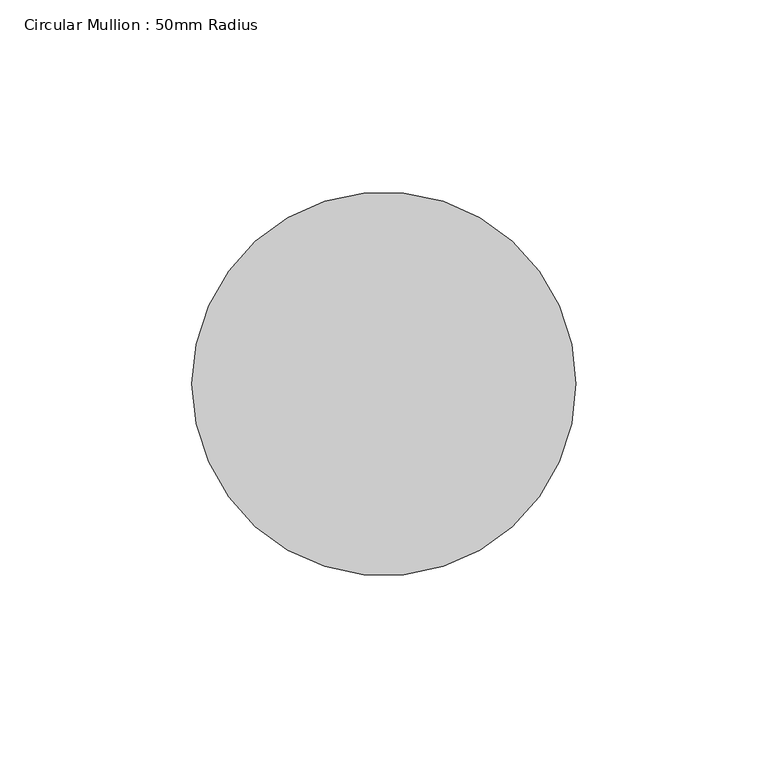
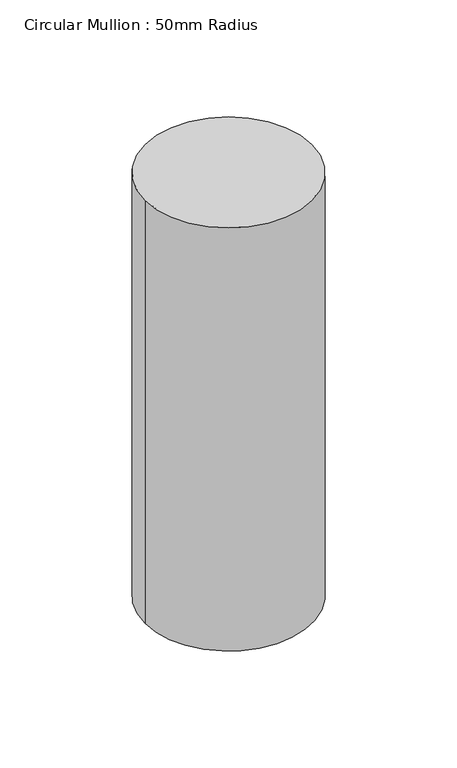
"""IFC4 building model written with IfcOpenShell, lengths in millimetres: member geometry, Circular Mullion : 50mm Radius."""

import ifcopenshell
import ifcopenshell.guid

model = None  # the IFC model being written
_history = None  # IfcOwnerHistory: only IFC2X3 demands one
_inside = {}  # id of a spatial element -> (the spatial element, [elements in it])
_under = {}  # id of a project, library or spatial element -> (it, [spatial elements below it])
_declared = {}  # id of a project -> (the project, [libraries it declares])
_typed = {}  # id of a type object -> (the type object, [elements of that type])
_made_of = {}  # id of a material, layer set ... -> (it, [elements and type objects made of it])


def new_model(schema):
    """Start an empty IFC model of exactly this schema.

    Asked for "IFC4X3", IfcOpenShell would pick the latest addendum, in which some entities
    have other attributes; the version numbers below select the first issue.
    IFC2X3 requires an IfcOwnerHistory on every rooted entity: one is made here for all.
    """
    global model, _history
    if schema == "IFC4X3":
        model = ifcopenshell.file(schema_version=(4, 3, 0, 0))
    else:
        model = ifcopenshell.file(schema=schema)
    _inside.clear()
    _under.clear()
    _declared.clear()
    _typed.clear()
    _made_of.clear()
    _history = None
    if model.schema == "IFC2X3":
        org = make("IfcOrganization", Name="unknown")
        user = make(
            "IfcPersonAndOrganization",
            ThePerson=make("IfcPerson", FamilyName="unknown"),
            TheOrganization=org,
        )
        app = make(
            "IfcApplication",
            ApplicationDeveloper=org,
            Version="unknown",
            ApplicationFullName="unknown",
            ApplicationIdentifier="unknown",
        )
        _history = make(
            "IfcOwnerHistory",
            OwningUser=user,
            OwningApplication=app,
            ChangeAction="ADDED",
            CreationDate=0,
        )
    return model


def make(cls, **values):
    """One entity of the class cls with the attributes given. An attribute that is None is left unset."""
    return model.create_entity(
        cls, **{name: value for name, value in values.items() if value is not None}
    )


def rooted(cls, **values):
    """An entity with a GlobalId (a new one), such as an element, a storey or a relation."""
    return make(cls, GlobalId=ifcopenshell.guid.new(), OwnerHistory=_history, **values)


def si_unit(unit_type, name, prefix=None):
    """IfcSIUnit, for example si_unit("LENGTHUNIT", "METRE", prefix="MILLI")."""
    return make("IfcSIUnit", UnitType=unit_type, Prefix=prefix, Name=name)


def assignment(units):
    """IfcUnitAssignment: the units of a project."""
    return None if units is None else make("IfcUnitAssignment", Units=units)


def point(xyz):
    """IfcCartesianPoint."""
    return None if xyz is None else make("IfcCartesianPoint", Coordinates=xyz)


def direction(xyz):
    """IfcDirection."""
    return None if xyz is None else make("IfcDirection", DirectionRatios=xyz)


def frame(location, z_axis=None, x_axis=None):
    """IfcAxis2Placement3D, a coordinate frame: its origin and axes. An axis left out is left unset."""
    return make(
        "IfcAxis2Placement3D",
        Location=point(location),
        Axis=direction(z_axis),
        RefDirection=direction(x_axis),
    )


def frame_2d(location, x_axis=None):
    """IfcAxis2Placement2D, a coordinate frame in the plane: its origin and x axis."""
    return make(
        "IfcAxis2Placement2D", Location=point(location), RefDirection=direction(x_axis)
    )


def origin():
    """The frame at (0, 0, 0) with its axes left unset."""
    return frame((0.0, 0.0, 0.0))


def origin_2d():
    """The frame at (0, 0) in the plane with its x axis left unset."""
    return frame_2d((0.0, 0.0))


def place(relative_to, where):
    """IfcLocalPlacement: puts the frame where relative to a parent placement (None: the world)."""
    return make(
        "IfcLocalPlacement", PlacementRelTo=relative_to, RelativePlacement=where
    )


def context(
    kind, dimensions, precision=None, world=None, true_north=None, identifier=None
):
    """IfcGeometricRepresentationContext, for example the 3D "Model" context."""
    return make(
        "IfcGeometricRepresentationContext",
        ContextIdentifier=identifier,
        ContextType=kind,
        CoordinateSpaceDimension=dimensions,
        Precision=precision,
        WorldCoordinateSystem=world,
        TrueNorth=true_north,
    )


def project(units=None, contexts=None):
    """IfcProject with its units and contexts."""
    return rooted(
        "IfcProject",
        Name="project",
        RepresentationContexts=contexts,
        UnitsInContext=assignment(units),
    )


def spatial(cls, under=None, at=None, **own):
    """A site, building, storey or space (cls), placed at a placement, below another one or the project."""
    s = rooted(cls, ObjectPlacement=at, **own)
    if under is not None:
        _under.setdefault(under.id(), (under, []))[1].append(s)
    return s


def circle_curve(where, radius):
    """IfcCircle in the frame where."""
    return make("IfcCircle", Position=where, Radius=radius)


def trimmed(basis, trim1, trim2, sense, master):
    """IfcTrimmedCurve: the piece of a basis curve between two trims."""
    return make(
        "IfcTrimmedCurve",
        BasisCurve=basis,
        Trim1=trim1,
        Trim2=trim2,
        SenseAgreement=sense,
        MasterRepresentation=master,
    )


def segment(curve, same_sense, transition):
    """IfcCompositeCurveSegment."""
    return make(
        "IfcCompositeCurveSegment",
        Transition=transition,
        SameSense=same_sense,
        ParentCurve=curve,
    )


def composite_curve(segments, self_intersect=None):
    """IfcCompositeCurve: segments joined end to end."""
    return make("IfcCompositeCurve", Segments=segments, SelfIntersect=self_intersect)


def outline(outer, holes=None, kind="AREA"):
    """IfcArbitraryClosedProfileDef: a profile drawn as a closed curve; with holes, ...WithVoids."""
    if holes is None:
        return make("IfcArbitraryClosedProfileDef", ProfileType=kind, OuterCurve=outer)
    return make(
        "IfcArbitraryProfileDefWithVoids",
        ProfileType=kind,
        OuterCurve=outer,
        InnerCurves=holes,
    )


def extrude(swept, where, along, depth):
    """IfcExtrudedAreaSolid: the profile swept, set in the frame where, extruded along a direction by depth."""
    return make(
        "IfcExtrudedAreaSolid",
        SweptArea=swept,
        Position=where,
        ExtrudedDirection=direction(along),
        Depth=depth,
    )


def shape(context_of_items, identifier, shape_type, items):
    """IfcShapeRepresentation: the items that make up one representation, for example the "Body"."""
    return make(
        "IfcShapeRepresentation",
        ContextOfItems=context_of_items,
        RepresentationIdentifier=identifier,
        RepresentationType=shape_type,
        Items=items,
    )


def source(mapping_origin, context_of_items, identifier, shape_type, items):
    """IfcRepresentationMap: a shape defined once, which mapped items show again and again."""
    return make(
        "IfcRepresentationMap",
        MappingOrigin=mapping_origin,
        MappedRepresentation=shape(context_of_items, identifier, shape_type, items),
    )


def transform(
    local_origin,
    x_axis=None,
    y_axis=None,
    z_axis=None,
    scale=None,
    scale2=None,
    scale3=None,
    uniform=True,
):
    """IfcCartesianTransformationOperator3D, or its non-uniform kind. x_axis, y_axis, z_axis: its Axis1, 2, 3."""
    if uniform:
        return make(
            "IfcCartesianTransformationOperator3D",
            Axis1=direction(x_axis),
            Axis2=direction(y_axis),
            LocalOrigin=point(local_origin),
            Scale=scale,
            Axis3=direction(z_axis),
        )
    return make(
        "IfcCartesianTransformationOperator3DnonUniform",
        Axis1=direction(x_axis),
        Axis2=direction(y_axis),
        LocalOrigin=point(local_origin),
        Scale=scale,
        Axis3=direction(z_axis),
        Scale2=scale2,
        Scale3=scale3,
    )


def mapped(mapping_source, mapping_target):
    """IfcMappedItem: shows the shape of a source again, moved by a transform."""
    return make(
        "IfcMappedItem", MappingSource=mapping_source, MappingTarget=mapping_target
    )


def made_of(thing, what):
    """Note that an element or type object is made of a material, layer set ...; save() writes the relation."""
    if what is not None:
        _made_of.setdefault(what.id(), (what, []))[1].append(thing)
    return thing


def element(
    cls,
    number,
    at=None,
    inside=None,
    cuts=None,
    type_object=None,
    material=None,
    context=None,
    identifier="Body",
    shape_type=None,
    held_by="IfcProductDefinitionShape",
    body=None,
    shapes=None,
    **own,
):
    """One element of the class cls, such as IfcWall. Its Tag is "e" and its number.

    at: its placement. inside: the storey or other place that contains it. cuts: it is an
    opening in that element (IfcRelVoidsElement). A single representation is given by context,
    identifier, shape_type and body (its items); several are given by shapes. held_by: the class
    of the entity that holds the representations. save() writes the other relations.
    """
    e = rooted(cls, Tag="e%d" % number, ObjectPlacement=at, **own)
    if body is not None:
        shapes = [shape(context, identifier, shape_type, body)]
    if shapes is not None:
        e.Representation = make(held_by, Representations=shapes)
    if inside is not None:
        _inside.setdefault(inside.id(), (inside, []))[1].append(e)
    if cuts is not None:
        rooted(
            "IfcRelVoidsElement", RelatingBuildingElement=cuts, RelatedOpeningElement=e
        )
    if type_object is not None:
        _typed.setdefault(type_object.id(), (type_object, []))[1].append(e)
    return made_of(e, material)


def aggregate(whole, parts):
    """IfcRelAggregates: a whole, such as a stair, and the parts it consists of."""
    return rooted("IfcRelAggregates", RelatingObject=whole, RelatedObjects=parts)


def save(model, path):
    """Write the relations noted so far, then the file.

    IfcRelAggregates (storeys below a building ...), IfcRelContainedInSpatialStructure (elements
    in a storey), IfcRelDefinesByType, IfcRelAssociatesMaterial and IfcRelDeclares: one each for
    every whole, place, type object, material and project.
    """
    for whole, parts in _under.values():
        aggregate(whole, parts)
    for where, things in _inside.values():
        rooted(
            "IfcRelContainedInSpatialStructure",
            RelatedElements=things,
            RelatingStructure=where,
        )
    for kind, things in _typed.values():
        rooted("IfcRelDefinesByType", RelatedObjects=things, RelatingType=kind)
    for what, things in _made_of.values():
        rooted("IfcRelAssociatesMaterial", RelatedObjects=things, RelatingMaterial=what)
    for by, libraries in _declared.values():
        rooted("IfcRelDeclares", RelatingContext=by, RelatedDefinitions=libraries)
    model.write(path)


def circular_mullion_50mm_radius_4487ff5f(model_context):
    return source(origin(), model_context, "Body", "SweptSolid", [
        extrude(outline(composite_curve([segment(trimmed(circle_curve(origin_2d(), 50.0), [point((50.0, 0.0))], [point((-50.0, 0.0))], False, "CARTESIAN"), True, "CONTINUOUS"), segment(trimmed(circle_curve(origin_2d(), 50.0), [point((-50.0, 0.0))], [point((50.0, 0.0))], False, "CARTESIAN"), True, "CONTINUOUS")], self_intersect=False)), frame((0.0, 0.0, -267.2084054), z_axis=(0.0, 0.0, 1.0), x_axis=(1.0, 0.0, 0.0)), (0.0, 0.0, 1.0), 267.2084054),
    ])


if __name__ == "__main__":
    model = new_model("IFC4")
    model_context = context("Model", 3, world=origin())
    ifc_project = project(units=[si_unit("LENGTHUNIT", "METRE", prefix="MILLI")], contexts=[model_context])
    site = spatial("IfcSite", under=ifc_project)
    building = spatial("IfcBuilding", under=site)
    placement = place(None, origin())
    circular_mullion_50mm_radius_shape = circular_mullion_50mm_radius_4487ff5f(model_context)
    element("IfcMember", 1, ObjectType="Circular Mullion : 50mm Radius", at=placement, inside=building, context=model_context, shape_type="MappedRepresentation", body=[
        mapped(circular_mullion_50mm_radius_shape, transform((0.0, 0.0, 0.0), x_axis=(1.0, 0.0, 0.0), y_axis=(0.0, 1.0, 0.0), z_axis=(0.0, 0.0, 1.0))),
    ])
    save(model, "model.ifc")

# Revit data of these elements
# Type "Circular Mullion : 50mm Radius"
#   built-in parameter 1007350 = 0.164042 (stored number, unit not read)
# Element 1 (IfcMember, "Circular Mullion : 50mm Radius")
#   Materials on its faces: "Aluminium"
# Materials
#   "Aluminium": class "Metal", colour RGB 247 247 247, transparency 0, Description = "Aluminium 6061", Cost = 0
